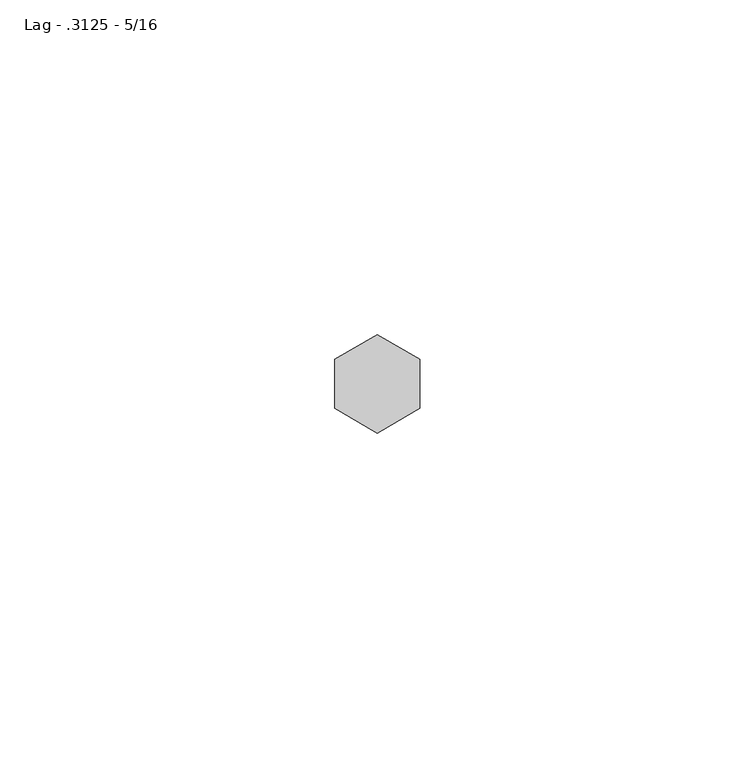
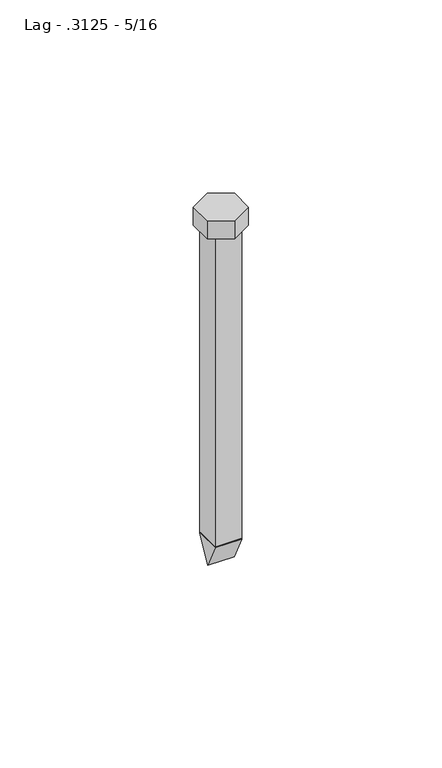
"""IFC4 building model written with IfcOpenShell, lengths in millimetres: fastener geometry, 060523 - W_P_C - Fastenings - Generic - SQUARE : Lag - .3125 - 5/16."""

import ifcopenshell
import ifcopenshell.guid

model = None  # the IFC model being written
_history = None  # IfcOwnerHistory: only IFC2X3 demands one
_inside = {}  # id of a spatial element -> (the spatial element, [elements in it])
_under = {}  # id of a project, library or spatial element -> (it, [spatial elements below it])
_declared = {}  # id of a project -> (the project, [libraries it declares])
_typed = {}  # id of a type object -> (the type object, [elements of that type])
_made_of = {}  # id of a material, layer set ... -> (it, [elements and type objects made of it])


def new_model(schema):
    """Start an empty IFC model of exactly this schema.

    Asked for "IFC4X3", IfcOpenShell would pick the latest addendum, in which some entities
    have other attributes; the version numbers below select the first issue.
    IFC2X3 requires an IfcOwnerHistory on every rooted entity: one is made here for all.
    """
    global model, _history
    if schema == "IFC4X3":
        model = ifcopenshell.file(schema_version=(4, 3, 0, 0))
    else:
        model = ifcopenshell.file(schema=schema)
    _inside.clear()
    _under.clear()
    _declared.clear()
    _typed.clear()
    _made_of.clear()
    _history = None
    if model.schema == "IFC2X3":
        org = make("IfcOrganization", Name="unknown")
        user = make(
            "IfcPersonAndOrganization",
            ThePerson=make("IfcPerson", FamilyName="unknown"),
            TheOrganization=org,
        )
        app = make(
            "IfcApplication",
            ApplicationDeveloper=org,
            Version="unknown",
            ApplicationFullName="unknown",
            ApplicationIdentifier="unknown",
        )
        _history = make(
            "IfcOwnerHistory",
            OwningUser=user,
            OwningApplication=app,
            ChangeAction="ADDED",
            CreationDate=0,
        )
    return model


def make(cls, **values):
    """One entity of the class cls with the attributes given. An attribute that is None is left unset."""
    return model.create_entity(
        cls, **{name: value for name, value in values.items() if value is not None}
    )


def rooted(cls, **values):
    """An entity with a GlobalId (a new one), such as an element, a storey or a relation."""
    return make(cls, GlobalId=ifcopenshell.guid.new(), OwnerHistory=_history, **values)


def si_unit(unit_type, name, prefix=None):
    """IfcSIUnit, for example si_unit("LENGTHUNIT", "METRE", prefix="MILLI")."""
    return make("IfcSIUnit", UnitType=unit_type, Prefix=prefix, Name=name)


def assignment(units):
    """IfcUnitAssignment: the units of a project."""
    return None if units is None else make("IfcUnitAssignment", Units=units)


def point(xyz):
    """IfcCartesianPoint."""
    return None if xyz is None else make("IfcCartesianPoint", Coordinates=xyz)


def direction(xyz):
    """IfcDirection."""
    return None if xyz is None else make("IfcDirection", DirectionRatios=xyz)


def frame(location, z_axis=None, x_axis=None):
    """IfcAxis2Placement3D, a coordinate frame: its origin and axes. An axis left out is left unset."""
    return make(
        "IfcAxis2Placement3D",
        Location=point(location),
        Axis=direction(z_axis),
        RefDirection=direction(x_axis),
    )


def origin():
    """The frame at (0, 0, 0) with its axes left unset."""
    return frame((0.0, 0.0, 0.0))


def origin_with_axes():
    """The frame at (0, 0, 0) with the z axis (0, 0, 1) and the x axis (1, 0, 0) written out."""
    return frame((0.0, 0.0, 0.0), z_axis=(0.0, 0.0, 1.0), x_axis=(1.0, 0.0, 0.0))


def place(relative_to, where):
    """IfcLocalPlacement: puts the frame where relative to a parent placement (None: the world)."""
    return make(
        "IfcLocalPlacement", PlacementRelTo=relative_to, RelativePlacement=where
    )


def context(
    kind, dimensions, precision=None, world=None, true_north=None, identifier=None
):
    """IfcGeometricRepresentationContext, for example the 3D "Model" context."""
    return make(
        "IfcGeometricRepresentationContext",
        ContextIdentifier=identifier,
        ContextType=kind,
        CoordinateSpaceDimension=dimensions,
        Precision=precision,
        WorldCoordinateSystem=world,
        TrueNorth=true_north,
    )


def project(units=None, contexts=None):
    """IfcProject with its units and contexts."""
    return rooted(
        "IfcProject",
        Name="project",
        RepresentationContexts=contexts,
        UnitsInContext=assignment(units),
    )


def spatial(cls, under=None, at=None, **own):
    """A site, building, storey or space (cls), placed at a placement, below another one or the project."""
    s = rooted(cls, ObjectPlacement=at, **own)
    if under is not None:
        _under.setdefault(under.id(), (under, []))[1].append(s)
    return s


def polyline(points):
    """IfcPolyline through the points."""
    return make("IfcPolyline", Points=[point(p) for p in points])


def outline(outer, holes=None, kind="AREA"):
    """IfcArbitraryClosedProfileDef: a profile drawn as a closed curve; with holes, ...WithVoids."""
    if holes is None:
        return make("IfcArbitraryClosedProfileDef", ProfileType=kind, OuterCurve=outer)
    return make(
        "IfcArbitraryProfileDefWithVoids",
        ProfileType=kind,
        OuterCurve=outer,
        InnerCurves=holes,
    )


def extrude(swept, where, along, depth):
    """IfcExtrudedAreaSolid: the profile swept, set in the frame where, extruded along a direction by depth."""
    return make(
        "IfcExtrudedAreaSolid",
        SweptArea=swept,
        Position=where,
        ExtrudedDirection=direction(along),
        Depth=depth,
    )


def shape(context_of_items, identifier, shape_type, items):
    """IfcShapeRepresentation: the items that make up one representation, for example the "Body"."""
    return make(
        "IfcShapeRepresentation",
        ContextOfItems=context_of_items,
        RepresentationIdentifier=identifier,
        RepresentationType=shape_type,
        Items=items,
    )


def source(mapping_origin, context_of_items, identifier, shape_type, items):
    """IfcRepresentationMap: a shape defined once, which mapped items show again and again."""
    return make(
        "IfcRepresentationMap",
        MappingOrigin=mapping_origin,
        MappedRepresentation=shape(context_of_items, identifier, shape_type, items),
    )


def transform(
    local_origin,
    x_axis=None,
    y_axis=None,
    z_axis=None,
    scale=None,
    scale2=None,
    scale3=None,
    uniform=True,
):
    """IfcCartesianTransformationOperator3D, or its non-uniform kind. x_axis, y_axis, z_axis: its Axis1, 2, 3."""
    if uniform:
        return make(
            "IfcCartesianTransformationOperator3D",
            Axis1=direction(x_axis),
            Axis2=direction(y_axis),
            LocalOrigin=point(local_origin),
            Scale=scale,
            Axis3=direction(z_axis),
        )
    return make(
        "IfcCartesianTransformationOperator3DnonUniform",
        Axis1=direction(x_axis),
        Axis2=direction(y_axis),
        LocalOrigin=point(local_origin),
        Scale=scale,
        Axis3=direction(z_axis),
        Scale2=scale2,
        Scale3=scale3,
    )


def mapped(mapping_source, mapping_target):
    """IfcMappedItem: shows the shape of a source again, moved by a transform."""
    return make(
        "IfcMappedItem", MappingSource=mapping_source, MappingTarget=mapping_target
    )


def made_of(thing, what):
    """Note that an element or type object is made of a material, layer set ...; save() writes the relation."""
    if what is not None:
        _made_of.setdefault(what.id(), (what, []))[1].append(thing)
    return thing


def element(
    cls,
    number,
    at=None,
    inside=None,
    cuts=None,
    type_object=None,
    material=None,
    context=None,
    identifier="Body",
    shape_type=None,
    held_by="IfcProductDefinitionShape",
    body=None,
    shapes=None,
    **own,
):
    """One element of the class cls, such as IfcWall. Its Tag is "e" and its number.

    at: its placement. inside: the storey or other place that contains it. cuts: it is an
    opening in that element (IfcRelVoidsElement). A single representation is given by context,
    identifier, shape_type and body (its items); several are given by shapes. held_by: the class
    of the entity that holds the representations. save() writes the other relations.
    """
    e = rooted(cls, Tag="e%d" % number, ObjectPlacement=at, **own)
    if body is not None:
        shapes = [shape(context, identifier, shape_type, body)]
    if shapes is not None:
        e.Representation = make(held_by, Representations=shapes)
    if inside is not None:
        _inside.setdefault(inside.id(), (inside, []))[1].append(e)
    if cuts is not None:
        rooted(
            "IfcRelVoidsElement", RelatingBuildingElement=cuts, RelatedOpeningElement=e
        )
    if type_object is not None:
        _typed.setdefault(type_object.id(), (type_object, []))[1].append(e)
    return made_of(e, material)


def aggregate(whole, parts):
    """IfcRelAggregates: a whole, such as a stair, and the parts it consists of."""
    return rooted("IfcRelAggregates", RelatingObject=whole, RelatedObjects=parts)


def save(model, path):
    """Write the relations noted so far, then the file.

    IfcRelAggregates (storeys below a building ...), IfcRelContainedInSpatialStructure (elements
    in a storey), IfcRelDefinesByType, IfcRelAssociatesMaterial and IfcRelDeclares: one each for
    every whole, place, type object, material and project.
    """
    for whole, parts in _under.values():
        aggregate(whole, parts)
    for where, things in _inside.values():
        rooted(
            "IfcRelContainedInSpatialStructure",
            RelatedElements=things,
            RelatingStructure=where,
        )
    for kind, things in _typed.values():
        rooted("IfcRelDefinesByType", RelatedObjects=things, RelatingType=kind)
    for what, things in _made_of.values():
        rooted("IfcRelAssociatesMaterial", RelatedObjects=things, RelatingMaterial=what)
    for by, libraries in _declared.values():
        rooted("IfcRelDeclares", RelatingContext=by, RelatedDefinitions=libraries)
    model.write(path)


def lag_3125_5_16_b9fc9e3e(model_context):
    return source(origin(), model_context, "Body", "SweptSolid", [
        extrude(outline(polyline([(0.0, -109.8296), (-4.1148, -101.6), (4.1148, -101.6), (0.0, -109.8296)])), frame((-4.1148, 0.0, 0.0), z_axis=(1.0, 0.0, 0.0), x_axis=(0.0, 1.0, 0.0)), (0.0, 0.0, 1.0), 8.2296),
        extrude(outline(polyline([(-6.35, 3.6661742), (0.0, 7.3323484), (6.35, 3.6661742), (6.35, -3.6661742), (0.0, -7.3323484), (-6.35, -3.6661742), (-6.35, 3.6661742)])), origin_with_axes(), (0.0, 0.0, 1.0), 5.953125),
        extrude(outline(polyline([(-4.1148, 4.1148), (4.1148, 4.1148), (4.1148, -4.1148), (-4.1148, -4.1148), (-4.1148, 4.1148)])), frame((0.0, 0.0, -101.6), z_axis=(0.0, 0.0, 1.0), x_axis=(1.0, 0.0, 0.0)), (0.0, 0.0, 1.0), 101.6),
    ])


if __name__ == "__main__":
    model = new_model("IFC4")
    model_context = context("Model", 3, world=origin())
    ifc_project = project(units=[si_unit("LENGTHUNIT", "METRE", prefix="MILLI")], contexts=[model_context])
    site = spatial("IfcSite", under=ifc_project)
    building = spatial("IfcBuilding", under=site)
    placement = place(None, origin())
    lag_3125_5_16_shape = lag_3125_5_16_b9fc9e3e(model_context)
    element("IfcFastener", 1, ObjectType="060523 - W_P_C - Fastenings - Generic - SQUARE : Lag - .3125 - 5/16", at=placement, inside=building, context=model_context, shape_type="MappedRepresentation", body=[
        mapped(lag_3125_5_16_shape, transform((0.0, 0.0, 0.0), x_axis=(1.0, 0.0, 0.0), y_axis=(0.0, 1.0, 0.0), z_axis=(0.0, 0.0, 1.0))),
    ])
    save(model, "model.ifc")

# Revit data of these elements
# Type "060523 - W_P_C - Fastenings - Generic - SQUARE : Lag - .3125 - 5/16"
#   Washer_Thickness = 0' - 0 5/64"
#   Washer Radius = 0' - 0.39638"
#   Washer Offset - Head = 0' - 0"
#   Washer Offset = 0' - 0"
#   Thickness_of_Substrate [instance default] = 0' - 1"
#   Side = 0' - 0 37/128"
#   Radius = 0' - 0.162"
#   Length [instance default] = 0' - 4"
#   Head Size = 0' - 0 1/2"
#   Head Radius = 0' - 0 1/4"
#   Head Height = 0' - 0 15/64"
#   Double Diameter = 0' - 0.648"
#   Diameter = 0' - 0.324"
#   Default Elevation = 4' - 0"
#   Washer_Nut_Visibility = no
#   Washer_Head_Visibility = no
#   Round_Head_Visibility = no
#   Point Visibility = yes
#   Nut_Visibility = no
#   Hex_Head_Visiblilty = yes
#   Washer Material = none
#   Bolt Material (Size) = AT SILL - FASTENER AT 24" O.C.
# Element 1 (IfcFastener, "060523 - W_P_C - Fastenings - Generic - SQUARE : Lag - .3125 - 5/16")
#   Materials on its faces: "AT SILL - FASTENER AT 24\" O.C."
# Materials
#   "AT SILL - FASTENER AT 24\" O.C.": class "Generic", colour RGB 120 120 120, transparency 0, Cost = 0
